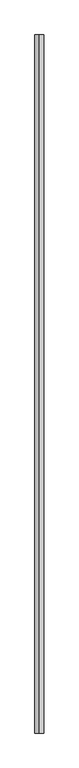
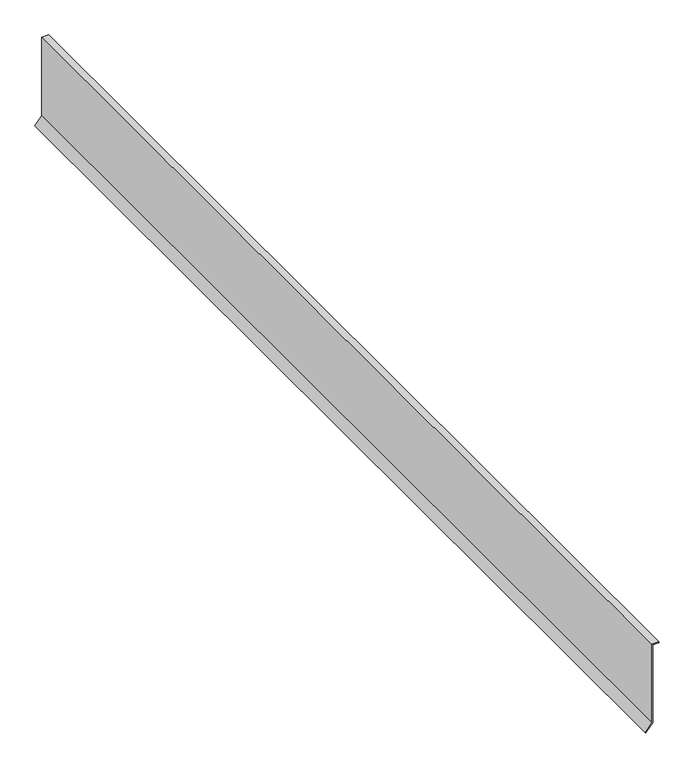
"""IFC4 building model written with IfcOpenShell, lengths in millimetres: proxy geometry, GRAVEL STOP001 4023 : GRAVEL STOP001 4023."""

from ifc_helpers import new_model, si_unit, frame, origin, place, context, project, spatial, polyline, outline, extrude, source, transform, mapped, element, save


def generic_models_e2b98164(model_context):
    return source(origin(), model_context, "Body", "SweptSolid", [
        extrude(outline(polyline([(40082.2407116, -2815.6343429), (40081.3605882, -2814.5313394), (40097.4918556, -2801.659661), (40253.3245993, -2801.659661), (40253.3245993, -2789.8917422), (40254.7357103, -2789.8917422), (40254.7357103, -2803.070772), (40097.9858473, -2803.070772), (40082.2407116, -2815.6343429)])), frame((0.0, -1052.8906573, 0.0), z_axis=(0.0, 1.0, 0.0), x_axis=(0.0, 0.0, 1.0)), (0.0, 0.0, 1.0), 2000.25),
    ])


if __name__ == "__main__":
    model = new_model("IFC4")
    model_context = context("Model", 3, world=origin())
    ifc_project = project(units=[si_unit("LENGTHUNIT", "METRE", prefix="MILLI")], contexts=[model_context])
    site = spatial("IfcSite", under=ifc_project)
    building = spatial("IfcBuilding", under=site)
    placement = place(None, origin())
    generic_models_shape = generic_models_e2b98164(model_context)
    element("IfcBuildingElementProxy", 1, Name="GRAVEL STOP001 4023 : GRAVEL STOP001 4023", ObjectType="GRAVEL STOP001 4023 : GRAVEL STOP001 4023", at=placement, inside=building, context=model_context, shape_type="MappedRepresentation", body=[
        mapped(generic_models_shape, transform((0.0, 0.0, 0.0), x_axis=(1.0, 0.0, 0.0), y_axis=(0.0, 1.0, 0.0), z_axis=(0.0, 0.0, 1.0))),
    ])
    save(model, "model.ifc")

# Revit data of these elements
# Type "GRAVEL STOP001 4023 : GRAVEL STOP001 4023"
#   NameOverride = "GRAVEL STOP001"
# Element 1 (IfcBuildingElementProxy, "GRAVEL STOP001 4023 : GRAVEL STOP001 4023")
#   Materials on its faces: "GRAVEL STOP REQUIRED WITH GRAVEL SURFACE SYSTEMS"
# Materials
#   "GRAVEL STOP REQUIRED WITH GRAVEL SURFACE SYSTEMS": class "Unassigned", colour RGB 170 170 127, transparency 0
